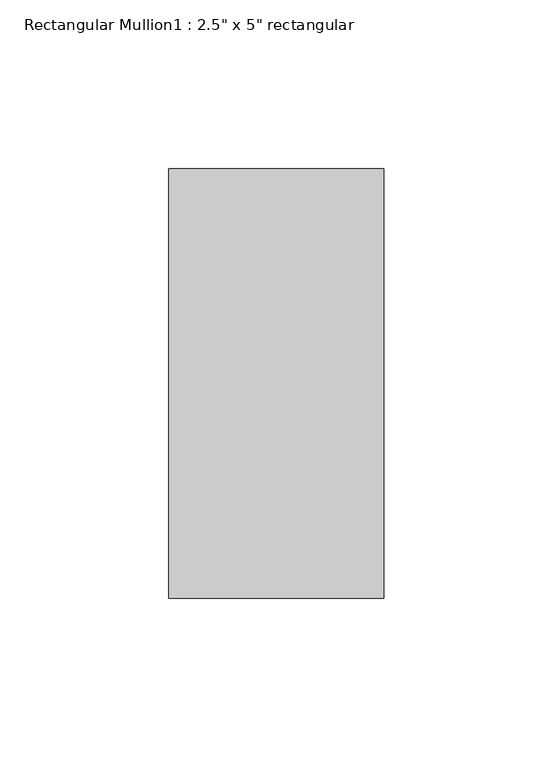
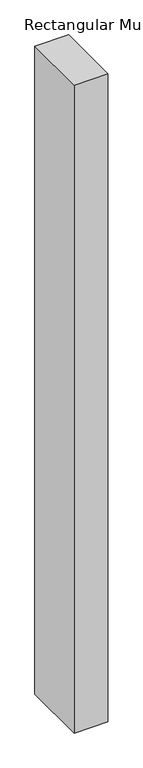
"""IFC4 building model written with IfcOpenShell, lengths in millimetres: member geometry."""

from ifc_helpers import new_model, si_unit, frame, origin, place, context, project, spatial, polyline, outline, extrude, source, transform, mapped, element, save


def member_98b79ab6(model_context):
    return source(origin(), model_context, "Body", "SweptSolid", [
        extrude(outline(polyline([(31.75, 63.5), (31.75, -63.5), (-31.75, -63.5), (-31.75, 63.5), (31.75, 63.5)])), frame((0.0, 0.0, -1282.7), z_axis=(0.0, 0.0, 1.0), x_axis=(1.0, 0.0, 0.0)), (0.0, 0.0, 1.0), 1282.7),
    ])


if __name__ == "__main__":
    model = new_model("IFC4")
    model_context = context("Model", 3, world=origin())
    ifc_project = project(units=[si_unit("LENGTHUNIT", "METRE", prefix="MILLI")], contexts=[model_context])
    site = spatial("IfcSite", under=ifc_project)
    building = spatial("IfcBuilding", under=site)
    placement = place(None, origin())
    member_shape = member_98b79ab6(model_context)
    element("IfcMember", 1, ObjectType="Rectangular Mullion1 : 2.5\" x 5\" rectangular", at=placement, inside=building, context=model_context, shape_type="MappedRepresentation", body=[
        mapped(member_shape, transform((0.0, 0.0, 0.0), x_axis=(1.0, 0.0, 0.0), y_axis=(0.0, 1.0, 0.0), z_axis=(0.0, 0.0, 1.0))),
    ])
    save(model, "model.ifc")

# Revit data of these elements
# Type "Rectangular Mullion1 : 2.5\" x 5\" rectangular"
#   built-in parameter 1007304 = 0.416667 (stored number, unit not read)
#   built-in parameter 1007301 = 0.104167 (stored number, unit not read)
#   built-in parameter 1007300 = 0.104167 (stored number, unit not read)
# Element 1 (IfcMember, "Rectangular Mullion1 : 2.5\" x 5\" rectangular")
#   Materials on its faces: "support-frame"
# Materials
#   "support-frame": class "Unassigned", colour RGB 233 233 233, transparency 0, Cost = 0
